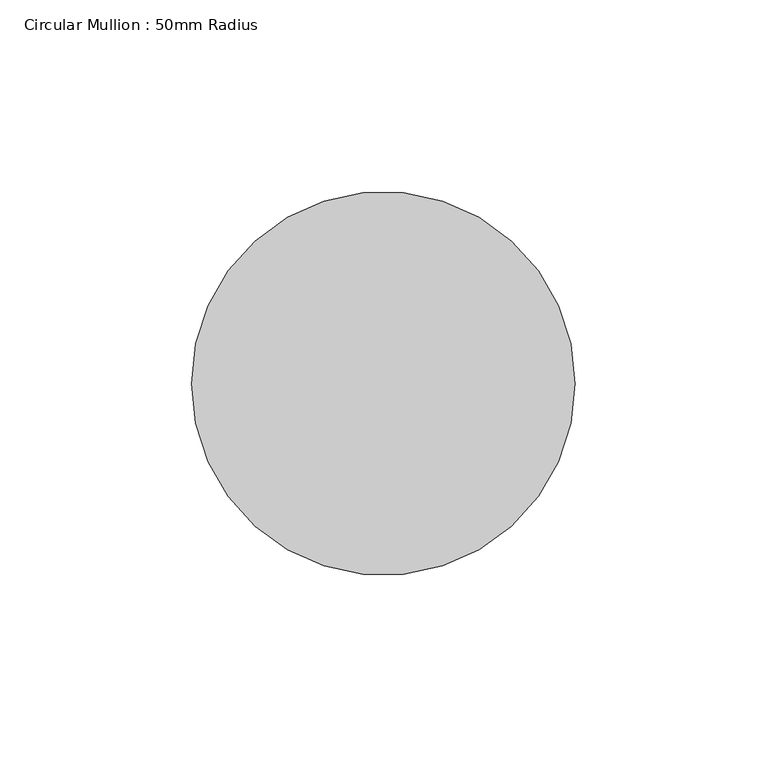
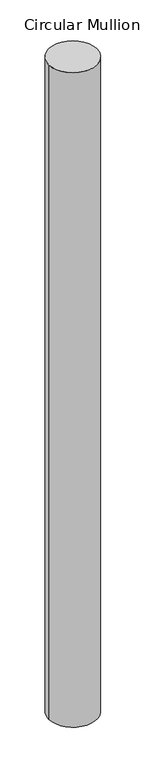
"""IFC4 building model written with IfcOpenShell, lengths in millimetres: member geometry, Circular Mullion : 50mm Radius."""

import ifcopenshell
import ifcopenshell.guid

model = None  # the IFC model being written
_history = None  # IfcOwnerHistory: only IFC2X3 demands one
_inside = {}  # id of a spatial element -> (the spatial element, [elements in it])
_under = {}  # id of a project, library or spatial element -> (it, [spatial elements below it])
_declared = {}  # id of a project -> (the project, [libraries it declares])
_typed = {}  # id of a type object -> (the type object, [elements of that type])
_made_of = {}  # id of a material, layer set ... -> (it, [elements and type objects made of it])


def new_model(schema):
    """Start an empty IFC model of exactly this schema.

    Asked for "IFC4X3", IfcOpenShell would pick the latest addendum, in which some entities
    have other attributes; the version numbers below select the first issue.
    IFC2X3 requires an IfcOwnerHistory on every rooted entity: one is made here for all.
    """
    global model, _history
    if schema == "IFC4X3":
        model = ifcopenshell.file(schema_version=(4, 3, 0, 0))
    else:
        model = ifcopenshell.file(schema=schema)
    _inside.clear()
    _under.clear()
    _declared.clear()
    _typed.clear()
    _made_of.clear()
    _history = None
    if model.schema == "IFC2X3":
        org = make("IfcOrganization", Name="unknown")
        user = make(
            "IfcPersonAndOrganization",
            ThePerson=make("IfcPerson", FamilyName="unknown"),
            TheOrganization=org,
        )
        app = make(
            "IfcApplication",
            ApplicationDeveloper=org,
            Version="unknown",
            ApplicationFullName="unknown",
            ApplicationIdentifier="unknown",
        )
        _history = make(
            "IfcOwnerHistory",
            OwningUser=user,
            OwningApplication=app,
            ChangeAction="ADDED",
            CreationDate=0,
        )
    return model


def make(cls, **values):
    """One entity of the class cls with the attributes given. An attribute that is None is left unset."""
    return model.create_entity(
        cls, **{name: value for name, value in values.items() if value is not None}
    )


def rooted(cls, **values):
    """An entity with a GlobalId (a new one), such as an element, a storey or a relation."""
    return make(cls, GlobalId=ifcopenshell.guid.new(), OwnerHistory=_history, **values)


def si_unit(unit_type, name, prefix=None):
    """IfcSIUnit, for example si_unit("LENGTHUNIT", "METRE", prefix="MILLI")."""
    return make("IfcSIUnit", UnitType=unit_type, Prefix=prefix, Name=name)


def assignment(units):
    """IfcUnitAssignment: the units of a project."""
    return None if units is None else make("IfcUnitAssignment", Units=units)


def point(xyz):
    """IfcCartesianPoint."""
    return None if xyz is None else make("IfcCartesianPoint", Coordinates=xyz)


def direction(xyz):
    """IfcDirection."""
    return None if xyz is None else make("IfcDirection", DirectionRatios=xyz)


def frame(location, z_axis=None, x_axis=None):
    """IfcAxis2Placement3D, a coordinate frame: its origin and axes. An axis left out is left unset."""
    return make(
        "IfcAxis2Placement3D",
        Location=point(location),
        Axis=direction(z_axis),
        RefDirection=direction(x_axis),
    )


def frame_2d(location, x_axis=None):
    """IfcAxis2Placement2D, a coordinate frame in the plane: its origin and x axis."""
    return make(
        "IfcAxis2Placement2D", Location=point(location), RefDirection=direction(x_axis)
    )


def origin():
    """The frame at (0, 0, 0) with its axes left unset."""
    return frame((0.0, 0.0, 0.0))


def origin_2d():
    """The frame at (0, 0) in the plane with its x axis left unset."""
    return frame_2d((0.0, 0.0))


def place(relative_to, where):
    """IfcLocalPlacement: puts the frame where relative to a parent placement (None: the world)."""
    return make(
        "IfcLocalPlacement", PlacementRelTo=relative_to, RelativePlacement=where
    )


def context(
    kind, dimensions, precision=None, world=None, true_north=None, identifier=None
):
    """IfcGeometricRepresentationContext, for example the 3D "Model" context."""
    return make(
        "IfcGeometricRepresentationContext",
        ContextIdentifier=identifier,
        ContextType=kind,
        CoordinateSpaceDimension=dimensions,
        Precision=precision,
        WorldCoordinateSystem=world,
        TrueNorth=true_north,
    )


def project(units=None, contexts=None):
    """IfcProject with its units and contexts."""
    return rooted(
        "IfcProject",
        Name="project",
        RepresentationContexts=contexts,
        UnitsInContext=assignment(units),
    )


def spatial(cls, under=None, at=None, **own):
    """A site, building, storey or space (cls), placed at a placement, below another one or the project."""
    s = rooted(cls, ObjectPlacement=at, **own)
    if under is not None:
        _under.setdefault(under.id(), (under, []))[1].append(s)
    return s


def circle_curve(where, radius):
    """IfcCircle in the frame where."""
    return make("IfcCircle", Position=where, Radius=radius)


def trimmed(basis, trim1, trim2, sense, master):
    """IfcTrimmedCurve: the piece of a basis curve between two trims."""
    return make(
        "IfcTrimmedCurve",
        BasisCurve=basis,
        Trim1=trim1,
        Trim2=trim2,
        SenseAgreement=sense,
        MasterRepresentation=master,
    )


def segment(curve, same_sense, transition):
    """IfcCompositeCurveSegment."""
    return make(
        "IfcCompositeCurveSegment",
        Transition=transition,
        SameSense=same_sense,
        ParentCurve=curve,
    )


def composite_curve(segments, self_intersect=None):
    """IfcCompositeCurve: segments joined end to end."""
    return make("IfcCompositeCurve", Segments=segments, SelfIntersect=self_intersect)


def outline(outer, holes=None, kind="AREA"):
    """IfcArbitraryClosedProfileDef: a profile drawn as a closed curve; with holes, ...WithVoids."""
    if holes is None:
        return make("IfcArbitraryClosedProfileDef", ProfileType=kind, OuterCurve=outer)
    return make(
        "IfcArbitraryProfileDefWithVoids",
        ProfileType=kind,
        OuterCurve=outer,
        InnerCurves=holes,
    )


def extrude(swept, where, along, depth):
    """IfcExtrudedAreaSolid: the profile swept, set in the frame where, extruded along a direction by depth."""
    return make(
        "IfcExtrudedAreaSolid",
        SweptArea=swept,
        Position=where,
        ExtrudedDirection=direction(along),
        Depth=depth,
    )


def shape(context_of_items, identifier, shape_type, items):
    """IfcShapeRepresentation: the items that make up one representation, for example the "Body"."""
    return make(
        "IfcShapeRepresentation",
        ContextOfItems=context_of_items,
        RepresentationIdentifier=identifier,
        RepresentationType=shape_type,
        Items=items,
    )


def source(mapping_origin, context_of_items, identifier, shape_type, items):
    """IfcRepresentationMap: a shape defined once, which mapped items show again and again."""
    return make(
        "IfcRepresentationMap",
        MappingOrigin=mapping_origin,
        MappedRepresentation=shape(context_of_items, identifier, shape_type, items),
    )


def transform(
    local_origin,
    x_axis=None,
    y_axis=None,
    z_axis=None,
    scale=None,
    scale2=None,
    scale3=None,
    uniform=True,
):
    """IfcCartesianTransformationOperator3D, or its non-uniform kind. x_axis, y_axis, z_axis: its Axis1, 2, 3."""
    if uniform:
        return make(
            "IfcCartesianTransformationOperator3D",
            Axis1=direction(x_axis),
            Axis2=direction(y_axis),
            LocalOrigin=point(local_origin),
            Scale=scale,
            Axis3=direction(z_axis),
        )
    return make(
        "IfcCartesianTransformationOperator3DnonUniform",
        Axis1=direction(x_axis),
        Axis2=direction(y_axis),
        LocalOrigin=point(local_origin),
        Scale=scale,
        Axis3=direction(z_axis),
        Scale2=scale2,
        Scale3=scale3,
    )


def mapped(mapping_source, mapping_target):
    """IfcMappedItem: shows the shape of a source again, moved by a transform."""
    return make(
        "IfcMappedItem", MappingSource=mapping_source, MappingTarget=mapping_target
    )


def made_of(thing, what):
    """Note that an element or type object is made of a material, layer set ...; save() writes the relation."""
    if what is not None:
        _made_of.setdefault(what.id(), (what, []))[1].append(thing)
    return thing


def element(
    cls,
    number,
    at=None,
    inside=None,
    cuts=None,
    type_object=None,
    material=None,
    context=None,
    identifier="Body",
    shape_type=None,
    held_by="IfcProductDefinitionShape",
    body=None,
    shapes=None,
    **own,
):
    """One element of the class cls, such as IfcWall. Its Tag is "e" and its number.

    at: its placement. inside: the storey or other place that contains it. cuts: it is an
    opening in that element (IfcRelVoidsElement). A single representation is given by context,
    identifier, shape_type and body (its items); several are given by shapes. held_by: the class
    of the entity that holds the representations. save() writes the other relations.
    """
    e = rooted(cls, Tag="e%d" % number, ObjectPlacement=at, **own)
    if body is not None:
        shapes = [shape(context, identifier, shape_type, body)]
    if shapes is not None:
        e.Representation = make(held_by, Representations=shapes)
    if inside is not None:
        _inside.setdefault(inside.id(), (inside, []))[1].append(e)
    if cuts is not None:
        rooted(
            "IfcRelVoidsElement", RelatingBuildingElement=cuts, RelatedOpeningElement=e
        )
    if type_object is not None:
        _typed.setdefault(type_object.id(), (type_object, []))[1].append(e)
    return made_of(e, material)


def aggregate(whole, parts):
    """IfcRelAggregates: a whole, such as a stair, and the parts it consists of."""
    return rooted("IfcRelAggregates", RelatingObject=whole, RelatedObjects=parts)


def save(model, path):
    """Write the relations noted so far, then the file.

    IfcRelAggregates (storeys below a building ...), IfcRelContainedInSpatialStructure (elements
    in a storey), IfcRelDefinesByType, IfcRelAssociatesMaterial and IfcRelDeclares: one each for
    every whole, place, type object, material and project.
    """
    for whole, parts in _under.values():
        aggregate(whole, parts)
    for where, things in _inside.values():
        rooted(
            "IfcRelContainedInSpatialStructure",
            RelatedElements=things,
            RelatingStructure=where,
        )
    for kind, things in _typed.values():
        rooted("IfcRelDefinesByType", RelatedObjects=things, RelatingType=kind)
    for what, things in _made_of.values():
        rooted("IfcRelAssociatesMaterial", RelatedObjects=things, RelatingMaterial=what)
    for by, libraries in _declared.values():
        rooted("IfcRelDeclares", RelatingContext=by, RelatedDefinitions=libraries)
    model.write(path)


def circular_mullion_50mm_radius_322dd969(model_context):
    return source(origin(), model_context, "Body", "SweptSolid", [
        extrude(outline(composite_curve([segment(trimmed(circle_curve(origin_2d(), 50.0), [point((50.0, 0.0))], [point((-50.0, 0.0))], False, "CARTESIAN"), True, "CONTINUOUS"), segment(trimmed(circle_curve(origin_2d(), 50.0), [point((-50.0, 0.0))], [point((50.0, 0.0))], False, "CARTESIAN"), True, "CONTINUOUS")], self_intersect=False)), frame((0.0, 0.0, -1429.9906179), z_axis=(0.0, 0.0, 1.0), x_axis=(1.0, 0.0, 0.0)), (0.0, 0.0, 1.0), 1429.9906179),
    ])


if __name__ == "__main__":
    model = new_model("IFC4")
    model_context = context("Model", 3, world=origin())
    ifc_project = project(units=[si_unit("LENGTHUNIT", "METRE", prefix="MILLI")], contexts=[model_context])
    site = spatial("IfcSite", under=ifc_project)
    building = spatial("IfcBuilding", under=site)
    placement = place(None, origin())
    circular_mullion_50mm_radius_shape = circular_mullion_50mm_radius_322dd969(model_context)
    element("IfcMember", 1, ObjectType="Circular Mullion : 50mm Radius", at=placement, inside=building, context=model_context, shape_type="MappedRepresentation", body=[
        mapped(circular_mullion_50mm_radius_shape, transform((0.0, 0.0, 0.0), x_axis=(1.0, 0.0, 0.0), y_axis=(0.0, 1.0, 0.0), z_axis=(0.0, 0.0, 1.0))),
    ])
    save(model, "model.ifc")

# Revit data of these elements
# Type "Circular Mullion : 50mm Radius"
#   built-in parameter 1007350 = 0.164042 (stored number, unit not read)
# Element 1 (IfcMember, "Circular Mullion : 50mm Radius")
#   Materials on its faces: "Aluminium"
# Materials
#   "Aluminium": class "Metal", colour RGB 247 247 247, transparency 0, Description = "Aluminium 6061", Cost = 0
